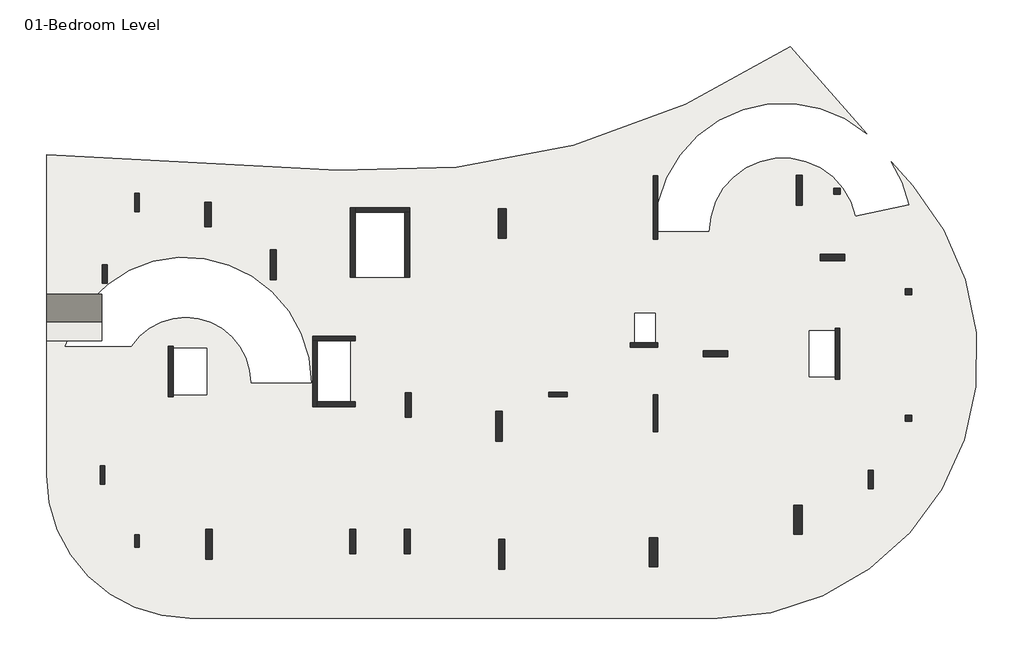
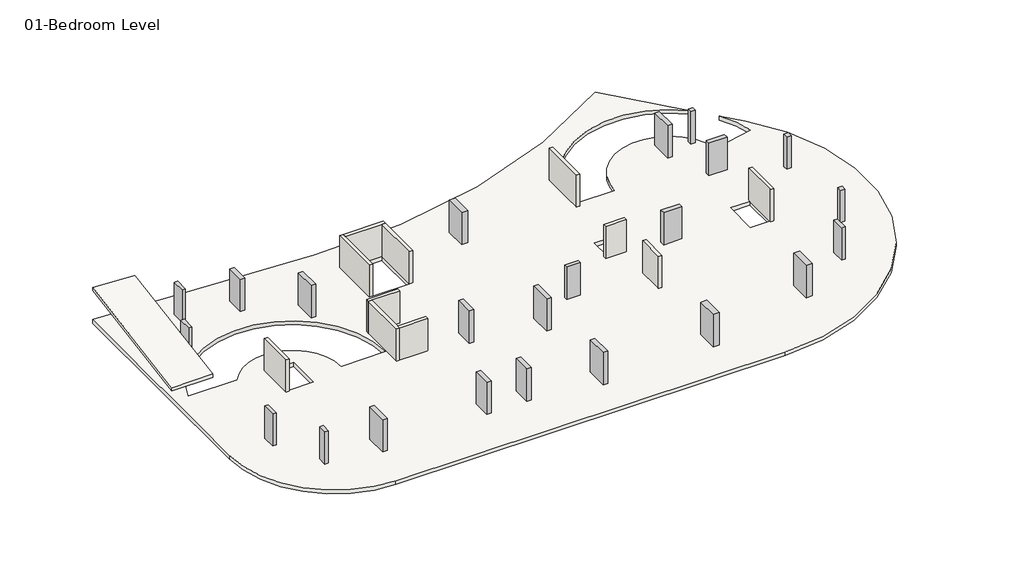
# One storey: 23 columns, 11 walls, 2 slabs.
"""IFC4 building model written with IfcOpenShell, lengths in millimetres."""

from ifc_helpers import new_model, si_unit, point, frame, frame_2d, origin, place, context, project, spatial, polyline, circle_curve, trimmed, segment, composite_curve, outline, extrude, faceted_brep, element, save

model = new_model("IFC4")

# Units and contexts
model_context = context("Model", 3, world=origin())
ifc_project = project(units=[si_unit("LENGTHUNIT", "METRE", prefix="MILLI")], contexts=[model_context])

# Site, building, storey
site = spatial("IfcSite", under=ifc_project)
building = spatial("IfcBuilding", under=site)
storey = spatial("IfcBuildingStorey", under=building, Name="01-Bedroom Level", Elevation=-3000.0)

# Columns
placement = place(None, origin())
element("IfcColumn", 1, ObjectType="M_Concrete-Rectangular-Column : C-1 (400 x 400mm)", at=placement, inside=storey, context=model_context, shape_type="Brep", body=[
    faceted_brep([(52549.9999998, 8504.0039609, -3000.0), (52549.9999998, 8104.0039609, -3000.0), (52149.9999998, 8104.0039609, -3000.0), (52149.9999998, 8504.0039609, -3000.0), (52549.9999998, 8504.0039609, 0.0), (52549.9999998, 8104.0039609, 0.0), (52549.9999998, 8104.0039609, -300.0), (52549.9999998, 8504.0039609, -300.0), (52149.9999998, 8104.0039609, 0.0), (52149.9999998, 8104.0039609, -300.0), (52149.9999998, 8504.0039609, 0.0), (52149.9999998, 8504.0039609, -300.0)], [[[0, 1, 2, 3]], [[4, 5, 6, 1, 0, 7]], [[5, 8, 9, 2, 1, 6]], [[8, 10, 11, 3, 2, 9]], [[10, 4, 7, 0, 3, 11]], [[4, 10, 8, 5]]]),
])
element("IfcColumn", 2, ObjectType="M_Concrete-Rectangular-Column : C-1 (400 x 400mm)", at=placement, inside=storey, context=model_context, shape_type="Brep", body=[
    faceted_brep([(47898.6337868, 23252.0, -3000.0), (47898.6337868, 22852.0, -3000.0), (47498.6337868, 22852.0, -3000.0), (47498.6337868, 23252.0, -3000.0), (47898.6337868, 23252.0, 0.0), (47898.6337868, 22852.0, 0.0), (47898.6337868, 22852.0, -300.0), (47898.6337868, 23252.0, -300.0), (47498.6337868, 22852.0, 0.0), (47498.6337868, 22852.0, -300.0), (47498.6337868, 23252.0, 0.0), (47498.6337868, 23252.0, -300.0)], [[[0, 1, 2, 3]], [[4, 5, 6, 1, 0, 7]], [[5, 8, 9, 2, 1, 6]], [[8, 10, 11, 3, 2, 9]], [[10, 4, 7, 0, 3, 11]], [[4, 10, 8, 5]]]),
])
element("IfcColumn", 3, ObjectType="M_Concrete-Rectangular-Column : C-1 (400 x 400mm)", at=placement, inside=storey, context=model_context, shape_type="Brep", body=[
    faceted_brep([(52549.9999998, 16712.0, -3000.0), (52549.9999998, 16312.0, -3000.0), (52149.9999998, 16312.0, -3000.0), (52149.9999998, 16712.0, -3000.0), (52549.9999998, 16712.0, 0.0), (52549.9999998, 16312.0, 0.0), (52549.9999998, 16312.0, -300.0), (52549.9999998, 16712.0, -300.0), (52149.9999998, 16312.0, 0.0), (52149.9999998, 16312.0, -300.0), (52149.9999998, 16712.0, 0.0), (52149.9999998, 16712.0, -300.0)], [[[0, 1, 2, 3]], [[4, 5, 6, 1, 0, 7]], [[5, 8, 9, 2, 1, 6]], [[8, 10, 11, 3, 2, 9]], [[10, 4, 7, 0, 3, 11]], [[4, 10, 8, 5]]]),
])
element("IfcColumn", 4, ObjectType="M_Concrete-Rectangular-Column : C-2 (300 x 800mm)", at=placement, inside=storey, context=model_context, shape_type="Brep", body=[
    faceted_brep([(2352.0, 728.0, -3000.0), (2352.0, -72.0, -3000.0), (2052.0, -72.0, -3000.0), (2052.0, 728.0, -3000.0), (2352.0, 728.0, 0.0), (2352.0, -72.0, 0.0), (2352.0, -72.0, -300.0), (2352.0, 728.0, -300.0), (2052.0, -72.0, 0.0), (2052.0, 728.0, 0.0)], [[[0, 1, 2, 3]], [[4, 5, 6, 1, 0, 7]], [[5, 8, 2, 1, 6]], [[8, 9, 3, 2]], [[9, 4, 7, 0, 3]], [[4, 9, 8, 5]]]),
])
element("IfcColumn", 5, ObjectType="M_Concrete-Rectangular-Column : C-3(300 x 1200mm)", at=placement, inside=storey, context=model_context, shape_type="SweptSolid", body=[
    extrude(outline(polyline([(2352.0, 22908.0000656), (2352.0, 21708.0000656), (2052.0, 21708.0000656), (2052.0, 22908.0000656), (2352.0, 22908.0000656)])), frame((0.0, 0.0, -3000.0), z_axis=(0.0, 0.0, 1.0), x_axis=(1.0, 0.0, 0.0)), (0.0, 0.0, 1.0), 3000.0),
])
element("IfcColumn", 6, ObjectType="M_Concrete-Rectangular-Column : C-3(300 x 1200mm)", at=placement, inside=storey, context=model_context, shape_type="SweptSolid", body=[
    extrude(outline(polyline([(257.9999999, 18288.0), (257.9999999, 17088.0), (-42.0000001, 17088.0), (-42.0000001, 18288.0), (257.9999999, 18288.0)])), frame((0.0, 0.0, -3000.0), z_axis=(0.0, 0.0, 1.0), x_axis=(1.0, 0.0, 0.0)), (0.0, 0.0, 1.0), 3000.0),
])
element("IfcColumn", 7, ObjectType="M_Concrete-Rectangular-Column : C-3(300 x 1200mm)", at=placement, inside=storey, context=model_context, shape_type="Brep", body=[
    faceted_brep([(108.001803, 5201.9999858, -3000.0), (108.001803, 4001.9999858, -3000.0), (-191.998197, 4001.9999858, -3000.0), (-191.998197, 5201.9999858, -3000.0), (108.001803, 5201.9999858, 0.0), (108.001803, 4001.9999858, 0.0), (108.001803, 4001.9999858, -300.0), (108.001803, 5201.9999858, -300.0), (-191.998197, 4001.9999858, 0.0), (-191.998197, 5201.9999858, 0.0), (-72.0008313, 5201.9999858, 0.0)], [[[0, 1, 2, 3]], [[4, 5, 6, 1, 0, 7]], [[5, 8, 2, 1, 6]], [[8, 9, 3, 2]], [[9, 10, 4, 7, 0, 3]], [[4, 10, 9, 8, 5]]]),
])
element("IfcColumn", 8, ObjectType="M_Concrete-Rectangular-Column : C-3(300 x 1200mm)", at=placement, inside=storey, context=model_context, shape_type="Brep", body=[
    faceted_brep([(50046.0009271, 4931.9999929, -3000.0), (50046.0009271, 3731.9999929, -3000.0), (49746.0009271, 3731.9999929, -3000.0), (49746.0009271, 4931.9999929, -3000.0), (50046.0009271, 4931.9999929, 0.0), (50046.0009271, 3731.9999929, 0.0), (50046.0009271, 3731.9999929, -300.0), (50046.0009271, 4931.9999929, -300.0), (49746.0009271, 3731.9999929, 0.0), (49746.0009271, 3731.9999929, -300.0), (49746.0009271, 4931.9999929, 0.0), (49746.0009271, 4931.9999929, -300.0)], [[[0, 1, 2, 3]], [[4, 5, 6, 1, 0, 7]], [[5, 8, 9, 2, 1, 6]], [[8, 10, 11, 3, 2, 9]], [[10, 4, 7, 0, 3, 11]], [[4, 10, 8, 5]]]),
])
element("IfcColumn", 9, ObjectType="M_Concrete-Rectangular-Column : C-3(300 x 1200mm)", at=placement, inside=storey, context=model_context, shape_type="SweptSolid", body=[
    extrude(outline(polyline([(28975.9999998, 9996.0000019), (30175.9999998, 9996.0000019), (30175.9999998, 9696.0000019), (28975.9999998, 9696.0000019), (28975.9999998, 9996.0000019)])), frame((0.0, 0.0, -3000.0), z_axis=(0.0, 0.0, 1.0), x_axis=(1.0, 0.0, 0.0)), (0.0, 0.0, 1.0), 3000.0),
])
element("IfcColumn", 10, ObjectType="M_Concrete-Rectangular-Column : C-4 (400 x 1600mm)", at=placement, inside=storey, context=model_context, shape_type="SweptSolid", body=[
    extrude(outline(polyline([(7021.9999999, 22340.0000078), (7021.9999999, 20740.0000078), (6621.9999999, 20740.0000078), (6621.9999999, 22340.0000078), (7021.9999999, 22340.0000078)])), frame((0.0, 0.0, -3000.0), z_axis=(0.0, 0.0, 1.0), x_axis=(1.0, 0.0, 0.0)), (0.0, 0.0, 1.0), 3000.0),
])
element("IfcColumn", 11, ObjectType="M_Concrete-Rectangular-Column : C-4 (400 x 1600mm)", at=placement, inside=storey, context=model_context, shape_type="SweptSolid", body=[
    extrude(outline(polyline([(19969.9997488, 1087.9955348), (19969.9997488, -512.0044652), (19569.9997488, -512.0044652), (19569.9997488, 1087.9955348), (19969.9997488, 1087.9955348)])), frame((0.0, 0.0, -3000.0), z_axis=(0.0, 0.0, 1.0), x_axis=(1.0, 0.0, 0.0)), (0.0, 0.0, 1.0), 3000.0),
])
element("IfcColumn", 12, ObjectType="M_Concrete-Rectangular-Column : C-4 (400 x 1600mm)", at=placement, inside=storey, context=model_context, shape_type="Brep", body=[
    faceted_brep([(46605.9993605, 18950.0, -3000.0), (48205.9993605, 18950.0, -3000.0), (48205.9993605, 18550.0, -3000.0), (46605.9993605, 18550.0, -3000.0), (46605.9993605, 18950.0, 0.0), (48205.9993605, 18950.0, 0.0), (48205.9993605, 18950.0, -300.0), (46605.9993605, 18950.0, -300.0), (48205.9993605, 18550.0, 0.0), (48205.9993605, 18550.0, -300.0), (46605.9993605, 18550.0, 0.0), (46605.9993605, 18550.0, -300.0)], [[[0, 1, 2, 3]], [[4, 5, 6, 1, 0, 7]], [[5, 8, 9, 2, 1, 6]], [[8, 10, 11, 3, 2, 9]], [[10, 4, 7, 0, 3, 11]], [[4, 10, 8, 5]]]),
])
element("IfcColumn", 13, ObjectType="M_Concrete-Rectangular-Column : C-5 (400 x 1600mm)", at=placement, inside=storey, context=model_context, shape_type="SweptSolid", body=[
    extrude(outline(polyline([(20030.000009, 9955.9999979), (20030.000009, 8355.9999979), (19630.000009, 8355.9999979), (19630.000009, 9955.9999979), (20030.000009, 9955.9999979)])), frame((0.0, 0.0, -3000.0), z_axis=(0.0, 0.0, 1.0), x_axis=(1.0, 0.0, 0.0)), (0.0, 0.0, 1.0), 3000.0),
])
element("IfcColumn", 14, ObjectType="M_Concrete-Rectangular-Column : C-5 (400 x 1600mm)", at=placement, inside=storey, context=model_context, shape_type="SweptSolid", body=[
    extrude(outline(polyline([(16429.9999981, 1088.0), (16429.9999981, -512.0), (16029.9999981, -512.0), (16029.9999981, 1088.0), (16429.9999981, 1088.0)])), frame((0.0, 0.0, -3000.0), z_axis=(0.0, 0.0, 1.0), x_axis=(1.0, 0.0, 0.0)), (0.0, 0.0, 1.0), 3000.0),
])
element("IfcColumn", 15, ObjectType="M_Concrete-Rectangular-Column : C-5 (400 x 1600mm)", at=placement, inside=storey, context=model_context, shape_type="Brep", body=[
    faceted_brep([(38998.0014887, 12692.0079212, -3000.0), (40598.0014887, 12692.0079212, -3000.0), (40598.0014887, 12292.0079212, -3000.0), (38998.0014887, 12292.0079212, -3000.0), (38998.0014887, 12692.0079212, 0.0), (40598.0014887, 12692.0079212, 0.0), (40598.0014887, 12692.0079212, -300.0), (38998.0014887, 12692.0079212, -300.0), (40598.0014887, 12292.0079212, 0.0), (40598.0014887, 12292.0079212, -300.0), (38998.0014887, 12292.0079212, 0.0), (38998.0014887, 12292.0079212, -300.0)], [[[0, 1, 2, 3]], [[4, 5, 6, 1, 0, 7]], [[5, 8, 9, 2, 1, 6]], [[8, 10, 11, 3, 2, 9]], [[10, 4, 7, 0, 3, 11]], [[4, 10, 8, 5]]]),
])
element("IfcColumn", 16, ObjectType="M_Concrete-Rectangular-Column : C-6 (400 x 1950mm)", at=placement, inside=storey, context=model_context, shape_type="SweptSolid", body=[
    extrude(outline(polyline([(11270.0000427, 19262.9999996), (11270.0000427, 17312.9999996), (10870.0000427, 17312.9999996), (10870.0000427, 19262.9999996), (11270.0000427, 19262.9999996)])), frame((0.0, 0.0, -3000.0), z_axis=(0.0, 0.0, 1.0), x_axis=(1.0, 0.0, 0.0)), (0.0, 0.0, 1.0), 3000.0),
])
element("IfcColumn", 17, ObjectType="M_Concrete-Rectangular-Column : C-6 (400 x 1950mm)", at=placement, inside=storey, context=model_context, shape_type="SweptSolid", body=[
    extrude(outline(polyline([(7082.0000416, 1083.0000153), (7082.0000416, -866.9999847), (6682.0000416, -866.9999847), (6682.0000416, 1083.0000153), (7082.0000416, 1083.0000153)])), frame((0.0, 0.0, -3000.0), z_axis=(0.0, 0.0, 1.0), x_axis=(1.0, 0.0, 0.0)), (0.0, 0.0, 1.0), 3000.0),
])
element("IfcColumn", 18, ObjectType="M_Concrete-Rectangular-Column : C-6 (400 x 1950mm)", at=placement, inside=storey, context=model_context, shape_type="SweptSolid", body=[
    extrude(outline(polyline([(26113.9999998, 422.995535), (26113.9999998, -1527.004465), (25713.9999998, -1527.004465), (25713.9999998, 422.995535), (26113.9999998, 422.995535)])), frame((0.0, 0.0, -3000.0), z_axis=(0.0, 0.0, 1.0), x_axis=(1.0, 0.0, 0.0)), (0.0, 0.0, 1.0), 3000.0),
])
element("IfcColumn", 19, ObjectType="M_Concrete-Rectangular-Column : C-6 (400 x 1950mm)", at=placement, inside=storey, context=model_context, shape_type="Brep", body=[
    faceted_brep([(45446.0007483, 24087.0, -3000.0), (45446.0007483, 22137.0, -3000.0), (45046.0007483, 22137.0, -3000.0), (45046.0007483, 24087.0, -3000.0), (45446.0007483, 24087.0, 0.0), (45446.0007483, 22137.0, 0.0), (45446.0007483, 22137.0, -300.0), (45446.0007483, 24087.0, -300.0), (45046.0007483, 22137.0, 0.0), (45046.0007483, 22137.0, -300.0), (45046.0007483, 24087.0, 0.0), (45046.0007483, 24087.0, -300.0)], [[[0, 1, 2, 3]], [[4, 5, 6, 1, 0, 7]], [[5, 8, 9, 2, 1, 6]], [[8, 10, 11, 3, 2, 9]], [[10, 4, 7, 0, 3, 11]], [[4, 10, 8, 5]]]),
])
element("IfcColumn", 20, ObjectType="M_Concrete-Rectangular-Column : C-6 (400 x 1950mm)", at=placement, inside=storey, context=model_context, shape_type="SweptSolid", body=[
    extrude(outline(polyline([(25934.0000455, 8751.0001824), (25934.0000455, 6801.0001824), (25534.0000455, 6801.0001824), (25534.0000455, 8751.0001824), (25934.0000455, 8751.0001824)])), frame((0.0, 0.0, -3000.0), z_axis=(0.0, 0.0, 1.0), x_axis=(1.0, 0.0, 0.0)), (0.0, 0.0, 1.0), 3000.0),
])
element("IfcColumn", 21, ObjectType="M_Concrete-Rectangular-Column : C-7 (550 x 1900mm)", at=placement, inside=storey, context=model_context, shape_type="SweptSolid", body=[
    extrude(outline(polyline([(36035.9999998, 548.0007983), (36035.9999998, -1351.9992017), (35485.9999998, -1351.9992017), (35485.9999998, 548.0007983), (36035.9999998, 548.0007983)])), frame((0.0, 0.0, -3000.0), z_axis=(0.0, 0.0, 1.0), x_axis=(1.0, 0.0, 0.0)), (0.0, 0.0, 1.0), 3000.0),
])
element("IfcColumn", 22, ObjectType="M_Concrete-Rectangular-Column : C-7 (550 x 1900mm)", at=placement, inside=storey, context=model_context, shape_type="Brep", body=[
    faceted_brep([(45443.9999998, 2648.0, -3000.0), (45443.9999998, 748.0, -3000.0), (44893.9999998, 748.0, -3000.0), (44893.9999998, 2648.0, -3000.0), (45443.9999998, 2648.0, 0.0), (45443.9999998, 748.0, 0.0), (45443.9999998, 748.0, -300.0), (45443.9999998, 2648.0, -300.0), (44893.9999998, 748.0, 0.0), (44893.9999998, 748.0, -300.0), (44893.9999998, 2648.0, 0.0), (44893.9999998, 2648.0, -300.0)], [[[0, 1, 2, 3]], [[4, 5, 6, 1, 0, 7]], [[5, 8, 9, 2, 1, 6]], [[8, 10, 11, 3, 2, 9]], [[10, 4, 7, 0, 3, 11]], [[4, 10, 8, 5]]]),
])
element("IfcColumn", 23, ObjectType="M_Concrete-Rectangular-Column : C-7 (550 x 1900mm)", at=placement, inside=storey, context=model_context, shape_type="SweptSolid", body=[
    extrude(outline(polyline([(26218.9999998, 21900.0), (26218.9999998, 20000.0), (25668.9999998, 20000.0), (25668.9999998, 21900.0), (26218.9999998, 21900.0)])), frame((0.0, 0.0, -3000.0), z_axis=(0.0, 0.0, 1.0), x_axis=(1.0, 0.0, 0.0)), (0.0, 0.0, 1.0), 3000.0),
])

# Slabs
element("IfcSlab", 24, ObjectType="Generic 300mm", at=placement, inside=storey, context=model_context, shape_type="Brep", body=[
    faceted_brep([(-72.0008313, 25234.895247, -320.2846119), (-72.0008313, 13331.7741591, -2304.1381265), (-3672.0008313, 13331.7741591, -2304.1381265), (-3672.0008313, 25428.6530713, -287.9916412), (-208.1213467, 25242.2214734, -319.0635741), (-72.0008313, 13331.7741591, -2000.0), (-72.0008313, 25234.895247, -16.1464854), (-208.1213467, 25242.2214734, -14.9254476), (-1872.0008313, 25331.7741591, 0.0), (-3672.0008313, 25428.6530713, 16.1464854), (-3672.0008313, 13331.7741591, -2000.0), (-3672.0008313, 25428.6530713, 0.0)], [[[0, 1, 2, 3, 4]], [[5, 6, 7, 8, 9, 10]], [[6, 0, 4, 3, 11, 9, 8, 7]], [[1, 0, 6, 5]], [[3, 2, 10, 9, 11]], [[2, 1, 5, 10]]]),
])
element("IfcSlab", 25, ObjectType="Generic 350mm", at=placement, inside=storey, context=model_context, shape_type="SweptSolid", body=[
    extrude(outline(composite_curve([segment(trimmed(circle_curve(frame_2d((39909.3379075, 12227.9999997)), 16919.9999999), [point((52613.9117742, 23402.9811122))], [point((39909.3379075, -4692.0000002))], False, "CARTESIAN"), True, "CONTINUOUS"), segment(polyline([(39909.3379075, -4692.0000002), (5628.0036678, -4692.0000002)]), True, "CONTINUOUS"), segment(trimmed(circle_curve(frame_2d((5628.0036678, 4608.0044989)), 9300.0044991), [point((5628.0036678, -4692.0000002))], [point((-3672.0008313, 4608.000071))], False, "CARTESIAN"), True, "CONTINUOUS"), segment(polyline([(-3672.0008313, 4608.000071), (-3672.0008313, 25428.6530713), (15256.5094829, 24409.8900228)]), True, "CONTINUOUS"), segment(trimmed(circle_curve(frame_2d((17852.3365926, 72640.0847329)), 48300.0000016), [point((15256.5094829, 24409.8900228))], [point((44650.6358236, 32456.2427254))], True, "CARTESIAN"), True, "CONTINUOUS"), segment(polyline([(44650.6358236, 32456.2427254), (49633.7745991, 26791.0291538)]), True, "CONTINUOUS"), segment(trimmed(circle_curve(frame_2d((44207.404779, 20412.0)), 8374.8135722), [point((49633.7745991, 26791.0291538))], [point((36047.9999998, 22299.2244217))], True, "CARTESIAN"), True, "CONTINUOUS"), segment(polyline([(36047.9999998, 22299.2244217), (36047.9999998, 24072.0078999), (35747.9999998, 24072.0078999), (35747.9999998, 19932.0), (36047.9999998, 19932.0), (36047.9999998, 20412.0), (39407.5912068, 20412.0)]), True, "CONTINUOUS"), segment(trimmed(circle_curve(frame_2d((44207.404779, 20412.0)), 4799.8135722), [point((39407.5912068, 20412.0))], [point((48900.364577, 21419.1438143))], False, "CARTESIAN"), True, "CONTINUOUS"), segment(polyline([(48900.364577, 21419.1438143), (52395.7776853, 22169.2852691)]), True, "CONTINUOUS"), segment(trimmed(circle_curve(frame_2d((44207.404779, 20412.0)), 8374.8135722), [point((52395.7776853, 22169.2852691))], [point((51226.6279201, 24980.1515809))], True, "CARTESIAN"), True, "CONTINUOUS"), segment(polyline([(51226.6279201, 24980.1515809), (52613.9117742, 23402.9811122)]), True, "CONTINUOUS")], self_intersect=False), holes=[polyline([(2352.0, 21708.0000656), (2352.0, 22908.0000656), (2052.0, 22908.0000656), (2052.0, 21708.0000656), (2352.0, 21708.0000656)]), polyline([(257.9999999, 17088.0), (257.9999999, 18288.0), (-42.0000001, 18288.0), (-42.0000001, 17088.0), (257.9999999, 17088.0)]), polyline([(108.001803, 4001.9999858), (108.001803, 5201.9999858), (-191.998197, 5201.9999858), (-191.998197, 4001.9999858), (108.001803, 4001.9999858)]), polyline([(50046.0009271, 3731.9999929), (50046.0009271, 4931.9999929), (49746.0009271, 4931.9999929), (49746.0009271, 3731.9999929), (50046.0009271, 3731.9999929)]), polyline([(30175.9999998, 9996.0000019), (28975.9999998, 9996.0000019), (28975.9999998, 9696.0000019), (30175.9999998, 9696.0000019), (30175.9999998, 9996.0000019)]), polyline([(7021.9999999, 20740.0000078), (7021.9999999, 22340.0000078), (6621.9999999, 22340.0000078), (6621.9999999, 20740.0000078), (7021.9999999, 20740.0000078)]), polyline([(19969.9997488, -512.0044652), (19969.9997488, 1087.9955348), (19569.9997488, 1087.9955348), (19569.9997488, -512.0044652), (19969.9997488, -512.0044652)]), polyline([(48205.9993605, 18950.0), (46605.9993605, 18950.0), (46605.9993605, 18550.0), (48205.9993605, 18550.0), (48205.9993605, 18950.0)]), polyline([(20030.000009, 8355.9999979), (20030.000009, 9955.9999979), (19630.000009, 9955.9999979), (19630.000009, 8355.9999979), (20030.000009, 8355.9999979)]), polyline([(16429.9999981, -512.0), (16429.9999981, 1088.0), (16029.9999981, 1088.0), (16029.9999981, -512.0), (16429.9999981, -512.0)]), polyline([(52549.9999998, 8104.0039609), (52549.9999998, 8504.0039609), (52149.9999998, 8504.0039609), (52149.9999998, 8104.0039609), (52549.9999998, 8104.0039609)]), polyline([(52549.9999998, 16312.0), (52549.9999998, 16712.0), (52149.9999998, 16712.0), (52149.9999998, 16312.0), (52549.9999998, 16312.0)]), polyline([(47898.6337868, 22852.0), (47898.6337868, 23252.0), (47498.6337868, 23252.0), (47498.6337868, 22852.0), (47898.6337868, 22852.0)]), polyline([(11270.0000427, 17312.9999996), (11270.0000427, 19262.9999996), (10870.0000427, 19262.9999996), (10870.0000427, 17312.9999996), (11270.0000427, 17312.9999996)]), polyline([(7082.0000416, -866.9999847), (7082.0000416, 1083.0000153), (6682.0000416, 1083.0000153), (6682.0000416, -866.9999847), (7082.0000416, -866.9999847)]), polyline([(26113.9999998, -1527.004465), (26113.9999998, 422.995535), (25713.9999998, 422.995535), (25713.9999998, -1527.004465), (26113.9999998, -1527.004465)]), polyline([(45446.0007483, 22137.0), (45446.0007483, 24087.0), (45046.0007483, 24087.0), (45046.0007483, 22137.0), (45446.0007483, 22137.0)]), polyline([(40598.0014887, 12692.0079212), (38998.0014887, 12692.0079212), (38998.0014887, 12292.0079212), (40598.0014887, 12292.0079212), (40598.0014887, 12692.0079212)]), polyline([(2352.0, -72.0), (2352.0, 728.0), (2052.0, 728.0), (2052.0, -72.0), (2352.0, -72.0)]), polyline([(25934.0000455, 6801.0001824), (25934.0000455, 8751.0001824), (25534.0000455, 8751.0001824), (25534.0000455, 6801.0001824), (25934.0000455, 6801.0001824)]), polyline([(36035.9999998, -1351.9992017), (36035.9999998, 548.0007983), (35485.9999998, 548.0007983), (35485.9999998, -1351.9992017), (36035.9999998, -1351.9992017)]), polyline([(45443.9999998, 748.0), (45443.9999998, 2648.0), (44893.9999998, 2648.0), (44893.9999998, 748.0), (45443.9999998, 748.0)]), polyline([(26218.9999998, 20000.0), (26218.9999998, 21900.0), (25668.9999998, 21900.0), (25668.9999998, 20000.0), (26218.9999998, 20000.0)]), polyline([(16079.9999907, 13320.0000002), (13919.9999907, 13320.0000002), (13919.9999907, 9359.999998), (16079.9999907, 9359.999998), (16079.9999907, 13320.0000002)]), polyline([(19619.9999997, 21672.0), (16379.9999997, 21672.0), (16379.9999997, 17468.0), (19619.9999997, 17468.0), (19619.9999997, 21672.0)]), polyline([(4548.0000034, 12840.0000003), (4548.0000034, 9840.0000003), (6743.9999995, 9840.0000003), (6743.9999995, 12840.0000003), (4548.0000034, 12840.0000003)]), polyline([(47580.0014798, 13992.0079177), (45900.001729, 13992.0079177), (45900.001729, 10992.0079181), (47580.0014798, 10992.0079181), (47580.0014798, 13992.0079177)]), polyline([(35904.002157, 15108.0000083), (34548.0015145, 15108.0000083), (34548.0015145, 13199.9999992), (35904.002157, 13199.9999992), (35904.002157, 15108.0000083)]), composite_curve([segment(polyline([(-2450.5143031, 12984.0000001), (1825.3666503, 12984.0000001)]), True, "CONTINUOUS"), segment(trimmed(circle_curve(frame_2d((5359.1233586, 10589.9997337)), 4268.3338376), [point((1825.3666503, 12984.0000001))], [point((9627.4571962, 10589.9997337))], False, "CARTESIAN"), True, "CONTINUOUS"), segment(polyline([(9627.4571962, 10589.9997337), (13527.4571962, 10589.9997337)]), True, "CONTINUOUS"), segment(trimmed(circle_curve(frame_2d((5359.1233586, 10589.9997337)), 8168.3338376), [point((13527.4571962, 10589.9997337))], [point((-2450.5143031, 12984.0000001))], True, "CARTESIAN"), True, "CONTINUOUS")], self_intersect=False)]), frame((0.0, 0.0, -3350.0), z_axis=(0.0, 0.0, 1.0), x_axis=(1.0, 0.0, 0.0)), (0.0, 0.0, 1.0), 350.0),
])

# Walls
element("IfcWall", 26, ObjectType="Shear Walls 300mm", at=placement, inside=storey, context=model_context, shape_type="Brep", body=[
    faceted_brep([(16379.9999997, 17468.0, -3000.0), (16379.9999997, 21672.0, -3000.0), (16379.9999997, 21972.0, -3000.0), (16379.9999997, 21972.0, 0.0), (16379.9999997, 21672.0, 0.0), (16379.9999997, 17468.0, 0.0), (16079.9999997, 17468.0, -3000.0), (16079.9999997, 17468.0, 0.0), (16079.9999997, 21972.0, 0.0), (16079.9999997, 21972.0, -3000.0)], [[[0, 1, 2, 3, 4, 5]], [[6, 7, 8, 9]], [[2, 1, 0, 6, 9]], [[5, 4, 3, 8, 7]], [[0, 5, 7, 6]], [[3, 2, 9, 8]]]),
])
element("IfcWall", 27, ObjectType="Shear Walls 300mm", at=placement, inside=storey, context=model_context, shape_type="Brep", body=[
    faceted_brep([(19919.9999997, 21972.0, -3000.0), (16379.9999997, 21972.0, -3000.0), (16379.9999997, 21972.0, -300.0), (16379.9999997, 21972.0, 0.0), (19919.9999997, 21972.0, 0.0), (19919.9999997, 21972.0, -300.0), (19919.9999997, 21672.0, -3000.0), (19919.9999997, 21672.0, 0.0), (19619.9999997, 21672.0, 0.0), (16379.9999997, 21672.0, 0.0), (16379.9999997, 21672.0, -3000.0), (19619.9999997, 21672.0, -3000.0)], [[[0, 1, 2, 3, 4, 5]], [[6, 7, 8, 9, 10, 11]], [[1, 0, 6, 11, 10]], [[4, 3, 9, 8, 7]], [[3, 2, 1, 10, 9]], [[0, 5, 4, 7, 6]]]),
])
element("IfcWall", 28, ObjectType="Shear Walls 300mm", at=placement, inside=storey, context=model_context, shape_type="Brep", body=[
    faceted_brep([(19919.9999997, 17468.0, -3000.0), (19919.9999997, 21672.0, -3000.0), (19919.9999997, 21672.0, 0.0), (19919.9999997, 17468.0, 0.0), (19919.9999997, 17468.0, -300.0), (19619.9999997, 17468.0, -3000.0), (19619.9999997, 17468.0, 0.0), (19619.9999997, 21672.0, 0.0), (19619.9999997, 21672.0, -3000.0)], [[[0, 1, 2, 3, 4]], [[5, 6, 7, 8]], [[1, 0, 5, 8]], [[3, 2, 7, 6]], [[0, 4, 3, 6, 5]], [[2, 1, 8, 7]]]),
])
element("IfcWall", 29, ObjectType="Shear Walls 300mm", at=placement, inside=storey, context=model_context, shape_type="Brep", body=[
    faceted_brep([(13619.9999907, 13320.0000002, -3000.0), (13919.9999907, 13320.0000002, -3000.0), (16380.0000168, 13320.0000002, -3000.0), (16380.0000168, 13320.0000002, 0.0), (13919.9999907, 13320.0000002, 0.0), (13619.9999907, 13320.0000002, 0.0), (13619.9999907, 13620.0000002, -3000.0), (13619.9999907, 13620.0000002, 0.0), (16380.0000168, 13620.0000002, 0.0), (16380.0000168, 13620.0000002, -3000.0)], [[[0, 1, 2, 3, 4, 5]], [[6, 7, 8, 9]], [[2, 1, 0, 6, 9]], [[3, 2, 9, 8]], [[5, 4, 3, 8, 7]], [[0, 5, 7, 6]]]),
])
element("IfcWall", 30, ObjectType="Shear Walls 300mm", at=placement, inside=storey, context=model_context, shape_type="Brep", body=[
    faceted_brep([(13919.9999907, 9059.999998, -3000.0), (13919.9999907, 9359.999998, -3000.0), (13919.9999907, 13320.0000002, -3000.0), (13919.9999907, 13320.0000002, 0.0), (13919.9999907, 9359.999998, 0.0), (13919.9999907, 9059.999998, 0.0), (13619.9999907, 9059.999998, -3000.0), (13619.9999907, 9059.999998, 0.0), (13619.9999907, 13320.0000002, 0.0), (13619.9999907, 13320.0000002, -3000.0)], [[[0, 1, 2, 3, 4, 5]], [[6, 7, 8, 9]], [[2, 1, 0, 6, 9]], [[5, 4, 3, 8, 7]], [[3, 2, 9, 8]], [[0, 5, 7, 6]]]),
])
element("IfcWall", 31, ObjectType="Shear Walls 300mm", at=placement, inside=storey, context=model_context, shape_type="SweptSolid", body=[
    extrude(outline(polyline([(13919.9999907, 9359.999998), (16380.0000168, 9359.999998), (16380.0000168, 9059.999998), (13919.9999907, 9059.999998), (13919.9999907, 9359.999998)])), frame((0.0, 0.0, -3000.0), z_axis=(0.0, 0.0, 1.0), x_axis=(1.0, 0.0, 0.0)), (0.0, 0.0, 1.0), 3000.0),
])
element("IfcWall", 32, ObjectType="Shear Walls 300mm", at=placement, inside=storey, context=model_context, shape_type="SweptSolid", body=[
    extrude(outline(polyline([(4548.0000025, 12984.0000001), (4548.0000025, 9696.0), (4248.0000025, 9696.0), (4248.0000025, 12984.0000001), (4548.0000025, 12984.0000001)])), frame((0.0, 0.0, -3000.0), z_axis=(0.0, 0.0, 1.0), x_axis=(1.0, 0.0, 0.0)), (0.0, 0.0, 1.0), 3000.0),
])
element("IfcWall", 33, ObjectType="Shear Walls 300mm", at=placement, inside=storey, context=model_context, shape_type="SweptSolid", body=[
    extrude(outline(polyline([(36048.0015201, 12899.9999992), (34248.0015201, 12899.9999992), (34248.0015201, 13199.9999992), (36048.0015201, 13199.9999992), (36048.0015201, 12899.9999992)])), frame((0.0, 0.0, -3000.0), z_axis=(0.0, 0.0, 1.0), x_axis=(1.0, 0.0, 0.0)), (0.0, 0.0, 1.0), 3000.0),
])
element("IfcWall", 34, ObjectType="Shear Walls 300mm", at=placement, inside=storey, context=model_context, shape_type="SweptSolid", body=[
    extrude(outline(polyline([(35748.0054035, 7428.0000762), (35748.0054035, 9840.0000002), (36048.0054035, 9840.0000002), (36048.0054035, 7428.0000762), (35748.0054035, 7428.0000762)])), frame((0.0, 0.0, -3000.0), z_axis=(0.0, 0.0, 1.0), x_axis=(1.0, 0.0, 0.0)), (0.0, 0.0, 1.0), 3000.0),
])
element("IfcWall", 35, ObjectType="Shear Walls 300mm", at=placement, inside=storey, context=model_context, shape_type="Brep", body=[
    faceted_brep([(47580.0014811, 14136.0000002, -3000.0), (47580.0014811, 10848.0079202, -3000.0), (47580.0014811, 10848.0079202, -300.0), (47580.0014811, 10848.0079202, 0.0), (47580.0014811, 10992.0079181, 0.0), (47580.0014811, 13992.0079177, 0.0), (47580.0014811, 14136.0000002, 0.0), (47580.0014811, 14136.0000002, -300.0), (47880.0014811, 10848.0079202, -3000.0), (47880.0014811, 14136.0000002, -3000.0), (47880.0014811, 14136.0000002, -300.0), (47880.0014811, 14136.0000002, 0.0), (47880.0014811, 10848.0079202, 0.0), (47880.0014811, 10848.0079202, -300.0)], [[[0, 1, 2, 3, 4, 5, 6, 7]], [[8, 9, 10, 11, 12, 13]], [[1, 0, 9, 8]], [[3, 2, 1, 8, 13, 12]], [[6, 5, 4, 3, 12, 11]], [[0, 7, 6, 11, 10, 9]]]),
])
element("IfcWall", 36, ObjectType="Shear Walls 300mm", at=placement, inside=storey, context=model_context, shape_type="SweptSolid", body=[
    extrude(outline(polyline([(36047.9999998, 24072.0078999), (36047.9999998, 19932.0), (35747.9999998, 19932.0), (35747.9999998, 24072.0078999), (36047.9999998, 24072.0078999)])), frame((0.0, 0.0, -3000.0), z_axis=(0.0, 0.0, 1.0), x_axis=(1.0, 0.0, 0.0)), (0.0, 0.0, 1.0), 3000.0),
])

save(model, "model.ifc")

# Revit data of these elements
# Project information
#   Project Issue Date = "Issue Date"
#   Project Status = "Project Status"
#   Client Name = "Owner"
#   Project Address = "Enter address here"
#   Project Name = "Project Name"
#   Project Number = "Project Number"
# Grids (mm)
#   "A": line (67449.899, 0) -> (-9043.592, 0)
#   "B": line (67449.899, 4800) -> (-9043.592, 4800)
#   "C": line (67449.899, 7896) -> (-9043.592, 7896)
#   "D": line (67449.899, 9924) -> (-9043.592, 9924)
#   "E": line (67449.899, 11418) -> (-9043.592, 11418)
#   "F": line (67449.899, 12756) -> (-9043.592, 12756)
#   "G": line (67449.899, 15900) -> (-9043.592, 15900)
#   "H": line (67449.899, 17400) -> (-9043.592, 17400)
#   "I": line (67449.899, 21900) -> (-9043.592, 21900)
#   "J": line (67449.899, 23160) -> (-9043.592, 23160)
#   "1": line (0, -11459.308) -> (0, 38805.288)
#   "2": line (2124, -11459.308) -> (2124, 38805.288)
#   "3": line (4320, -11459.308) -> (4320, 38805.288)
#   "4": line (6744, -11459.308) -> (6744, 38805.288)
#   "5": line (13848, -11459.308) -> (13848, 38805.288)
#   "6": line (16308, -11459.308) -> (16308, 38805.288)
#   "7": line (19692, -11459.308) -> (19692, 38805.288)
#   "8": line (25776, -11459.308) -> (25776, 38805.288)
#   "12": line (47808, -11459.308) -> (47808, 38805.288)
#   "13": line (50004, -11459.308) -> (50004, 38805.288)
#   "14": line (52428, -11459.308) -> (52428, 38805.288)
#   "9": line (35976, -11459.308) -> (35976, 38805.288)
#   "10": line (40068, -11459.308) -> (40068, 38805.288)
#   "11": line (45384, -11459.308) -> (45384, 38805.288)
# Type "M_Concrete-Rectangular-Column : C-1 (400 x 400mm)"
#   Type Mark = "C01"
#   b = 400 mm
#   h = 400 mm
#   Structural Material [instance default] = Concrete, Cast-in-Place gray
# Type "M_Concrete-Rectangular-Column : C-2 (300 x 800mm)"
#   Type Mark = "C02"
#   b = 300 mm
#   h = 800 mm
#   Structural Material [instance default] = Concrete, Cast-in-Place gray
# Type "M_Concrete-Rectangular-Column : C-3(300 x 1200mm)"
#   Type Mark = "C03"
#   b = 300 mm
#   h = 1200 mm
#   Structural Material [instance default] = Concrete, Cast-in-Place gray
# Type "M_Concrete-Rectangular-Column : C-4 (400 x 1600mm)"
#   Type Mark = "C04"
#   b = 400 mm
#   h = 1600 mm
#   Structural Material [instance default] = Concrete, Cast-in-Place gray
# Type "M_Concrete-Rectangular-Column : C-5 (400 x 1600mm)"
#   Type Mark = "C05"
#   b = 400 mm
#   h = 1600 mm
#   Structural Material [instance default] = Concrete, Cast-in-Place gray
# Type "M_Concrete-Rectangular-Column : C-6 (400 x 1950mm)"
#   Type Mark = "C06"
#   b = 400 mm
#   h = 1950 mm
#   Structural Material [instance default] = Concrete, Cast-in-Place gray
# Type "M_Concrete-Rectangular-Column : C-7 (550 x 1900mm)"
#   Type Mark = "C07"
#   b = 550 mm
#   h = 1900 mm
#   Structural Material [instance default] = Concrete, Cast-in-Place gray
# Type "Generic 300mm"
#   Function = 0
#   Layers, outside or top first: 300 mm "Concrete-RC" (function 1)
# Type "Generic 350mm"
#   Function = 0
#   Layers, outside or top first: 350 mm "Concrete-RC" (function 1)
# Type "Shear Walls 300mm"
#   Layers, outside or top first: 300 mm "Concrete-RC" (function 1)
# Elements 1, 2, 3 (IfcColumn, "M_Concrete-Rectangular-Column : C-1 (400 x 400mm)")
#   Structural Material = Concrete-RC
#   Phase Created = New Construction
#   Materials on its faces: "Concrete-RC"
# Element 4 (IfcColumn, "M_Concrete-Rectangular-Column : C-2 (300 x 800mm)")
#   Structural Material = Concrete-RC
#   Phase Created = New Construction
#   Materials on its faces: "Concrete-RC"
# Elements 5, 6, 7, 8, 9 (IfcColumn, "M_Concrete-Rectangular-Column : C-3(300 x 1200mm)")
#   Structural Material = Concrete-RC
#   Phase Created = New Construction
#   Materials on its faces: "Concrete-RC"
# Elements 10, 11, 12 (IfcColumn, "M_Concrete-Rectangular-Column : C-4 (400 x 1600mm)")
#   Structural Material = Concrete-RC
#   Phase Created = New Construction
#   Materials on its faces: "Concrete-RC"
# Elements 13, 14, 15 (IfcColumn, "M_Concrete-Rectangular-Column : C-5 (400 x 1600mm)")
#   Structural Material = Concrete-RC
#   Phase Created = New Construction
#   Materials on its faces: "Concrete-RC"
# Elements 16, 17, 18, 19, 20 (IfcColumn, "M_Concrete-Rectangular-Column : C-6 (400 x 1950mm)")
#   Structural Material = Concrete-RC
#   Phase Created = New Construction
#   Materials on its faces: "Concrete-RC"
# Elements 21, 22, 23 (IfcColumn, "M_Concrete-Rectangular-Column : C-7 (550 x 1900mm)")
#   Structural Material = Concrete-RC
#   Phase Created = New Construction
#   Materials on its faces: "Concrete-RC"
# Element 24 (IfcSlab, "Generic 300mm")
#   Height Offset From Level = 0 mm
#   built-in parameter 1001954 = 1
#   Phase Created = New Construction
#   Materials on its faces: "Concrete-RC"
# Element 25 (IfcSlab, "Generic 350mm")
#   built-in parameter 1001955 = -1.5708 (stored number, unit not read)
#   Height Offset From Level = 0 mm
#   built-in parameter 1001954 = 1
#   Phase Created = New Construction
#   Materials on its faces: "Concrete-RC"
# Elements 26, 27, 28, 29, 30, 31, 32, 33, 34, 35, 36 (IfcWall, "Shear Walls 300mm")
#   Top Offset = 0 mm
#   Base Offset = 0 mm
#   wall height = 3000 mm
#   Phase Created = New Construction
#   Base Constraint = 01-Bedroom Level
#   Top Constraint = 02-Ground Level
#   Materials on its faces: "Concrete-RC"
# Materials
#   "Concrete, Cast-in-Place gray": class "Concrete", colour RGB 192 192 192, transparency 0, Description = "Cast-in-place concrete", Cost = 0
#   "Concrete-RC": class "Concrete", colour RGB 128 128 128, transparency 0, Description = "High strength concrete", Cost = 0
